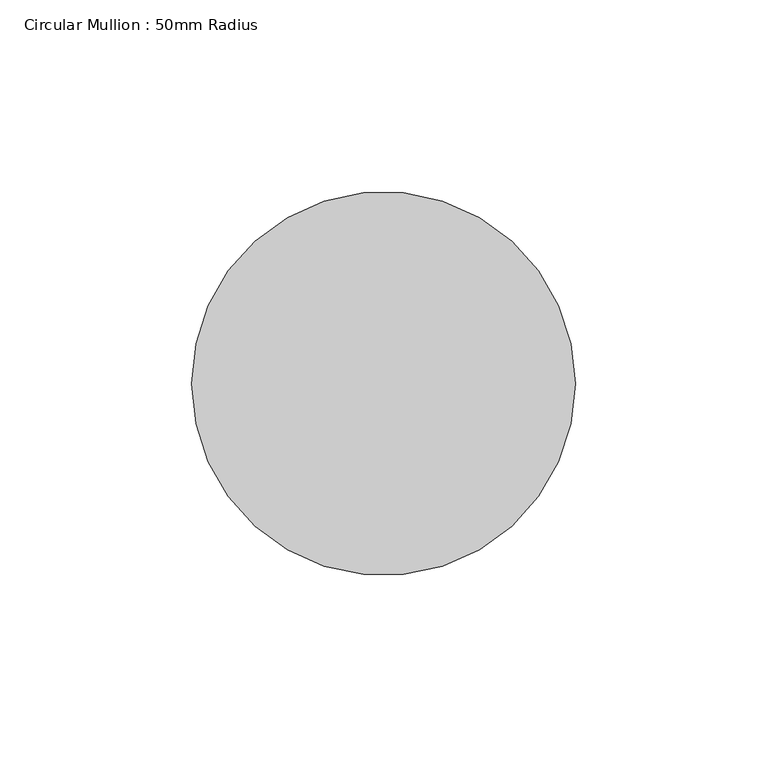
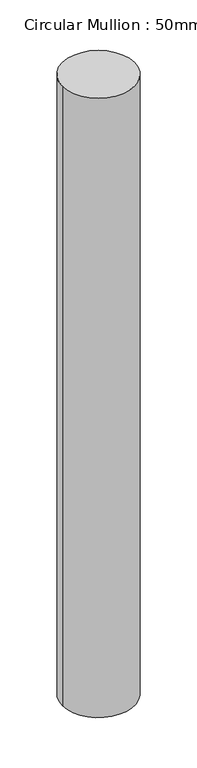
"""IFC4 building model written with IfcOpenShell, lengths in millimetres: member geometry, Circular Mullion : 50mm Radius."""

from ifc_helpers import new_model, si_unit, point, frame, origin, origin_2d, place, context, project, spatial, circle_curve, trimmed, segment, composite_curve, outline, extrude, source, transform, mapped, element, save


def circular_mullion_50mm_radius_3863e2a4(model_context):
    return source(origin(), model_context, "Body", "SweptSolid", [
        extrude(outline(composite_curve([segment(trimmed(circle_curve(origin_2d(), 50.0), [point((50.0, 0.0))], [point((-50.0, 0.0))], False, "CARTESIAN"), True, "CONTINUOUS"), segment(trimmed(circle_curve(origin_2d(), 50.0), [point((-50.0, 0.0))], [point((50.0, 0.0))], False, "CARTESIAN"), True, "CONTINUOUS")], self_intersect=False)), frame((0.0, 0.0, -906.7664046), z_axis=(0.0, 0.0, 1.0), x_axis=(1.0, 0.0, 0.0)), (0.0, 0.0, 1.0), 906.7664046),
    ])


if __name__ == "__main__":
    model = new_model("IFC4")
    model_context = context("Model", 3, world=origin())
    ifc_project = project(units=[si_unit("LENGTHUNIT", "METRE", prefix="MILLI")], contexts=[model_context])
    site = spatial("IfcSite", under=ifc_project)
    building = spatial("IfcBuilding", under=site)
    placement = place(None, origin())
    circular_mullion_50mm_radius_shape = circular_mullion_50mm_radius_3863e2a4(model_context)
    element("IfcMember", 1, ObjectType="Circular Mullion : 50mm Radius", at=placement, inside=building, context=model_context, shape_type="MappedRepresentation", body=[
        mapped(circular_mullion_50mm_radius_shape, transform((0.0, 0.0, 0.0), x_axis=(1.0, 0.0, 0.0), y_axis=(0.0, 1.0, 0.0), z_axis=(0.0, 0.0, 1.0))),
    ])
    save(model, "model.ifc")

# Revit data of these elements
# Type "Circular Mullion : 50mm Radius"
#   built-in parameter 1007350 = 0.164042 (stored number, unit not read)
# Element 1 (IfcMember, "Circular Mullion : 50mm Radius")
#   Materials on its faces: "Aluminium"
# Materials
#   "Aluminium": class "Metal", colour RGB 247 247 247, transparency 0, Description = "Aluminium 6061", Cost = 0
